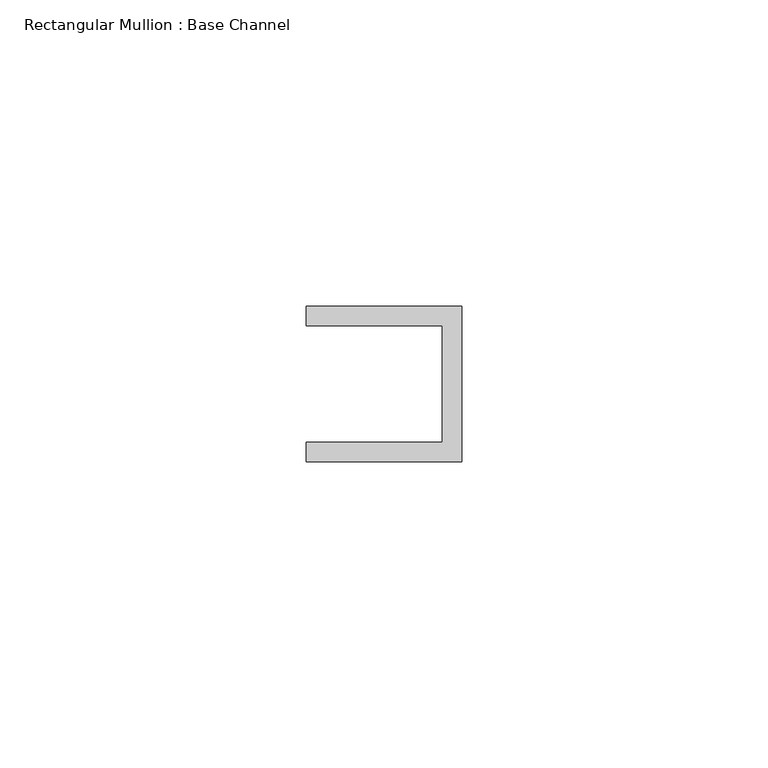
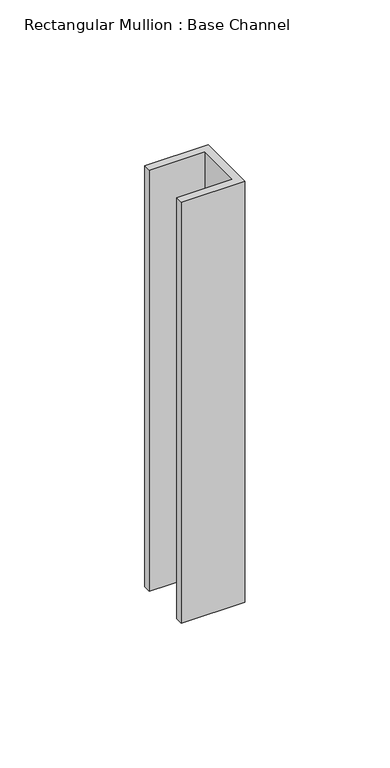
"""IFC4 building model written with IfcOpenShell, lengths in millimetres: member geometry, Rectangular Mullion : Base Channel."""

from ifc_helpers import new_model, si_unit, frame, origin, place, context, project, spatial, polyline, outline, extrude, source, transform, mapped, element, save


def rectangular_mullion_base_channel_59f3f779(model_context):
    return source(origin(), model_context, "Body", "SweptSolid", [
        extrude(outline(polyline([(0.0, -12.7), (-25.4, -12.7), (-25.4, -9.525), (-3.175, -9.525), (-3.175, 9.525), (-25.4, 9.525), (-25.4, 12.7), (0.0, 12.7), (0.0, -12.7)])), frame((0.0, 0.0, -177.8), z_axis=(0.0, 0.0, 1.0), x_axis=(1.0, 0.0, 0.0)), (0.0, 0.0, 1.0), 177.8),
    ])


if __name__ == "__main__":
    model = new_model("IFC4")
    model_context = context("Model", 3, world=origin())
    ifc_project = project(units=[si_unit("LENGTHUNIT", "METRE", prefix="MILLI")], contexts=[model_context])
    site = spatial("IfcSite", under=ifc_project)
    building = spatial("IfcBuilding", under=site)
    placement = place(None, origin())
    rectangular_mullion_base_channel_shape = rectangular_mullion_base_channel_59f3f779(model_context)
    element("IfcMember", 1, ObjectType="Rectangular Mullion : Base Channel", at=placement, inside=building, context=model_context, shape_type="MappedRepresentation", body=[
        mapped(rectangular_mullion_base_channel_shape, transform((0.0, 0.0, 0.0), x_axis=(1.0, 0.0, 0.0), y_axis=(0.0, 1.0, 0.0), z_axis=(0.0, 0.0, 1.0))),
    ])
    save(model, "model.ifc")

# Revit data of these elements
# Type "Rectangular Mullion : Base Channel"
#   built-in parameter 1007322 = 0.0833333 (stored number, unit not read)
#   built-in parameter 1007321 = 0.0416667 (stored number, unit not read)
#   built-in parameter 1007320 = -0.03125 (stored number, unit not read)
# Element 1 (IfcMember, "Rectangular Mullion : Base Channel")
#   Materials on its faces: "ALUM"
# Materials
#   "ALUM": class "Generic", colour RGB 157 157 157, transparency 0, Cost = 0
